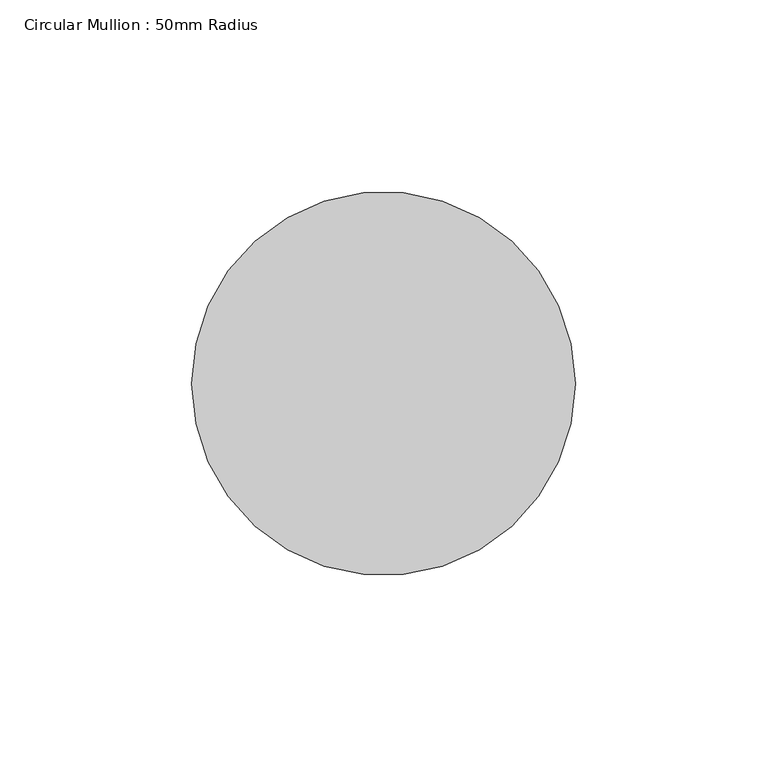
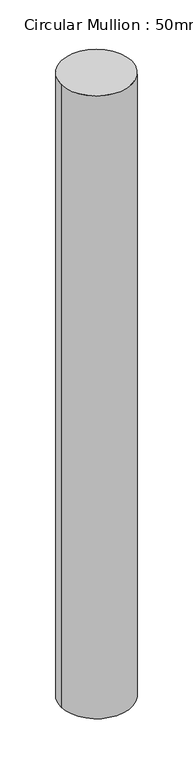
"""IFC4 building model written with IfcOpenShell, lengths in millimetres: member geometry, Circular Mullion : 50mm Radius."""

from ifc_helpers import new_model, si_unit, point, frame, origin, origin_2d, place, context, project, spatial, circle_curve, trimmed, segment, composite_curve, outline, extrude, source, transform, mapped, element, save


def circular_mullion_50mm_radius_872a91f8(model_context):
    return source(origin(), model_context, "Body", "SweptSolid", [
        extrude(outline(composite_curve([segment(trimmed(circle_curve(origin_2d(), 50.0), [point((50.0, 0.0))], [point((-50.0, 0.0))], False, "CARTESIAN"), True, "CONTINUOUS"), segment(trimmed(circle_curve(origin_2d(), 50.0), [point((-50.0, 0.0))], [point((50.0, 0.0))], False, "CARTESIAN"), True, "CONTINUOUS")], self_intersect=False)), frame((0.0, 0.0, -933.235457), z_axis=(0.0, 0.0, 1.0), x_axis=(1.0, 0.0, 0.0)), (0.0, 0.0, 1.0), 933.235457),
    ])


if __name__ == "__main__":
    model = new_model("IFC4")
    model_context = context("Model", 3, world=origin())
    ifc_project = project(units=[si_unit("LENGTHUNIT", "METRE", prefix="MILLI")], contexts=[model_context])
    site = spatial("IfcSite", under=ifc_project)
    building = spatial("IfcBuilding", under=site)
    placement = place(None, origin())
    circular_mullion_50mm_radius_shape = circular_mullion_50mm_radius_872a91f8(model_context)
    element("IfcMember", 1, ObjectType="Circular Mullion : 50mm Radius", at=placement, inside=building, context=model_context, shape_type="MappedRepresentation", body=[
        mapped(circular_mullion_50mm_radius_shape, transform((0.0, 0.0, 0.0), x_axis=(1.0, 0.0, 0.0), y_axis=(0.0, 1.0, 0.0), z_axis=(0.0, 0.0, 1.0))),
    ])
    save(model, "model.ifc")

# Revit data of these elements
# Type "Circular Mullion : 50mm Radius"
#   built-in parameter 1007350 = 0.164042 (stored number, unit not read)
# Element 1 (IfcMember, "Circular Mullion : 50mm Radius")
#   Materials on its faces: "Aluminium"
# Materials
#   "Aluminium": class "Metal", colour RGB 247 247 247, transparency 0, Description = "Aluminium 6061", Cost = 0
